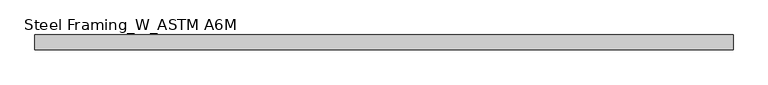
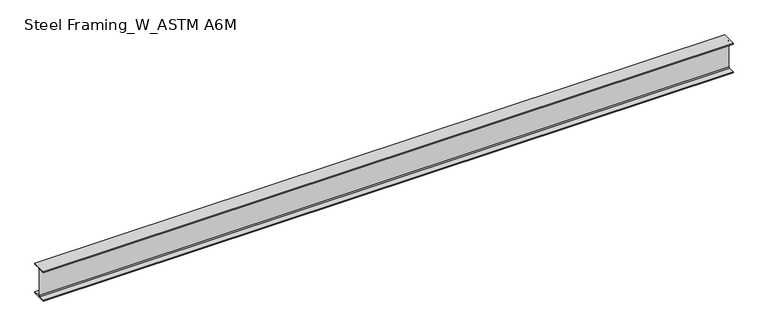
"""IFC4 building model written with IfcOpenShell, lengths in millimetres: beam geometry, Steel Framing_W_ASTM A6M : H_SB_AR_S02_W360x51_RB2."""

from ifc_helpers import new_model, si_unit, point, frame, frame_2d, origin, place, context, project, spatial, polyline, circle_curve, trimmed, segment, composite_curve, outline, extrude, source, transform, mapped, element, save


def steel_framing_w_astm_a6m_3dbe60e8(model_context):
    return source(origin(), model_context, "Body", "SweptSolid", [
        extrude(outline(composite_curve([segment(polyline([(85.5, -166.4), (85.5, -178.0), (-85.5, -178.0), (-85.5, -166.4), (-13.72, -166.4)]), True, "CONTINUOUS"), segment(trimmed(circle_curve(frame_2d((-13.72, -156.3)), 10.1), [point((-13.72, -166.4))], [point((-3.62, -156.3))], True, "CARTESIAN"), True, "CONTINUOUS"), segment(polyline([(-3.62, -156.3), (-3.62, 156.3)]), True, "CONTINUOUS"), segment(trimmed(circle_curve(frame_2d((-13.72, 156.3)), 10.1), [point((-3.62, 156.3))], [point((-13.72, 166.4))], True, "CARTESIAN"), True, "CONTINUOUS"), segment(polyline([(-13.72, 166.4), (-85.5, 166.4), (-85.5, 178.0), (85.5, 178.0), (85.5, 166.4), (13.72, 166.4)]), True, "CONTINUOUS"), segment(trimmed(circle_curve(frame_2d((13.72, 156.3)), 10.1), [point((13.72, 166.4))], [point((3.62, 156.3))], True, "CARTESIAN"), True, "CONTINUOUS"), segment(polyline([(3.62, 156.3), (3.62, -156.3)]), True, "CONTINUOUS"), segment(trimmed(circle_curve(frame_2d((13.72, -156.3)), 10.1), [point((3.62, -156.3))], [point((13.72, -166.4))], True, "CARTESIAN"), True, "CONTINUOUS"), segment(polyline([(13.72, -166.4), (85.5, -166.4)]), True, "CONTINUOUS")], self_intersect=False)), frame((-3879.15, 0.0, 0.0), z_axis=(1.0, 0.0, 0.0), x_axis=(0.0, 1.0, 0.0)), (0.0, 0.0, 1.0), 7939.9),
    ])


if __name__ == "__main__":
    model = new_model("IFC4")
    model_context = context("Model", 3, world=origin())
    ifc_project = project(units=[si_unit("LENGTHUNIT", "METRE", prefix="MILLI")], contexts=[model_context])
    site = spatial("IfcSite", under=ifc_project)
    building = spatial("IfcBuilding", under=site)
    placement = place(None, origin())
    steel_framing_w_astm_a6m_shape = steel_framing_w_astm_a6m_3dbe60e8(model_context)
    element("IfcBeam", 1, ObjectType="Steel Framing_W_ASTM A6M : H_SB_AR_S02_W360x51_RB2", at=placement, inside=building, context=model_context, shape_type="MappedRepresentation", body=[
        mapped(steel_framing_w_astm_a6m_shape, transform((0.0, 0.0, 0.0), x_axis=(1.0, 0.0, 0.0), y_axis=(0.0, 1.0, 0.0), z_axis=(0.0, 0.0, 1.0))),
    ])
    save(model, "model.ifc")

# Revit data of these elements
# Type "Steel Framing_W_ASTM A6M : H_SB_AR_S02_W360x51_RB2"
#   Type Mark = "RB2"
#   Section Name Key = "W14x34"
#   Width = 17.1 cm
#   Web Thickness = 0.724 cm
#   Web Fillet = 1.01 cm
#   Warping Constant = 287000.0 cm⁶
#   Torsional Moment of Inertia = 23.70 cm⁴
#   Section Area = 64.5 cm²
#   Plastic Modulus weak axis = 174.0 cm³
#   Plastic Modulus strong axis = 895.0 cm³
#   Perimeter = 1.36 m²/m
#   Nominal Weight = 51.00 kgf/m
#   Moment of Inertia weak axis = 970.00 cm⁴
#   Moment of Inertia strong axis = 14200.00 cm⁴
#   Height = 35.6 cm
#   Flange Thickness = 1.16 cm
#   Elastic Modulus weak axis = 113.0 cm³
#   Elastic Modulus strong axis = 796.0 cm³
#   Centroid Vertical = 17.8 cm
#   Centroid Horizontal = 8.55 cm
#   Length [instance default] = 1500 mm
#   Structural Material [instance default] = Steel, 45-345
#   Bolt Spacing = 0
#   Assembly Code = ""
# Element 1 (IfcBeam, "Steel Framing_W_ASTM A6M : H_SB_AR_S02_W360x51_RB2")
#   Materials on its faces: "Steel, 45-345"
# Materials
#   "Steel, 45-345": class "Metal", colour RGB 189 187 185, transparency 0, Description = "Steel 345 MPa", Cost = 0
